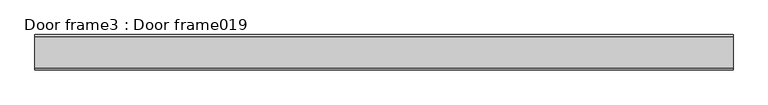
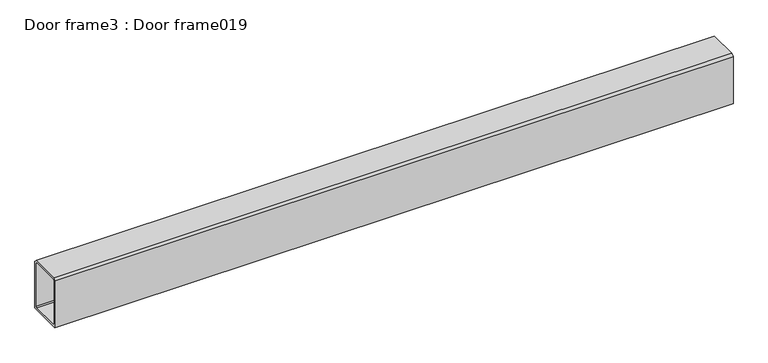
"""IFC4 building model written with IfcOpenShell, lengths in millimetres: proxy geometry, Door frame3 : Door frame019."""

from ifc_helpers import new_model, si_unit, frame, origin, place, context, project, spatial, polyline, outline, extrude, source, transform, mapped, element, save


def door_frame3_door_frame019_9a35ada2(model_context):
    return source(origin(), model_context, "Body", "SweptSolid", [
        extrude(outline(polyline([(9744.174946, 39528.496), (9750.524946, 39522.146), (9750.524946, 39376.096), (9648.924946, 39376.096), (9648.924946, 39522.146), (9655.274946, 39528.496), (9744.174946, 39528.496)]), holes=[polyline([(9744.174946, 39385.0762561), (9744.174946, 39519.5157439), (9741.5446899, 39522.146), (9657.9052021, 39522.146), (9655.274946, 39519.5157439), (9655.274946, 39385.0762561), (9657.9052021, 39382.446), (9741.5446899, 39382.446), (9744.174946, 39385.0762561)])]), frame((-9232.0719278, 0.0, 0.0), z_axis=(1.0, 0.0, 0.0), x_axis=(0.0, 1.0, 0.0)), (0.0, 0.0, 1.0), 1999.85),
    ])


if __name__ == "__main__":
    model = new_model("IFC4")
    model_context = context("Model", 3, world=origin())
    ifc_project = project(units=[si_unit("LENGTHUNIT", "METRE", prefix="MILLI")], contexts=[model_context])
    site = spatial("IfcSite", under=ifc_project)
    building = spatial("IfcBuilding", under=site)
    placement = place(None, origin())
    door_frame3_door_frame019_shape = door_frame3_door_frame019_9a35ada2(model_context)
    element("IfcBuildingElementProxy", 1, Name="Door frame3 : Door frame019", ObjectType="Door frame3 : Door frame019", at=placement, inside=building, context=model_context, shape_type="MappedRepresentation", body=[
        mapped(door_frame3_door_frame019_shape, transform((0.0, 0.0, 0.0), x_axis=(1.0, 0.0, 0.0), y_axis=(0.0, 1.0, 0.0), z_axis=(0.0, 0.0, 1.0))),
    ])
    save(model, "model.ifc")

# Revit data of these elements
# Type "Door frame3 : Door frame019"
#   NameOverride = "Door frame019"
# Element 1 (IfcBuildingElementProxy, "Door frame3 : Door frame019")
#   Materials on its faces: "DOOR FRAME: TUBE STEEL PROFILE - METALIZED, PRIMED & PAINTED (COLOR PER ARCHITECT)"
# Materials
#   "DOOR FRAME: TUBE STEEL PROFILE - METALIZED, PRIMED & PAINTED (COLOR PER ARCHITECT)": class "Unassigned", colour RGB 128 128 128, transparency 0, Cost = 0
